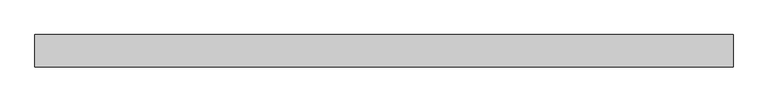
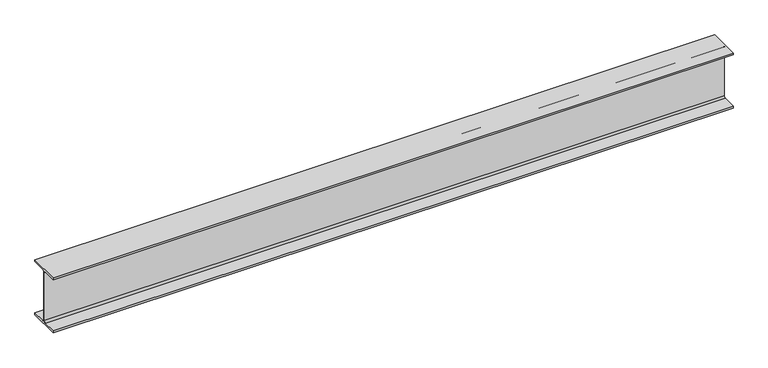
"""IFC4 building model written with IfcOpenShell, lengths in millimetres: beam geometry, Old_Steel Beam_H-KSD3502 : H_SB_ASB_H-200×200x8x12."""

from ifc_helpers import new_model, si_unit, point, frame, frame_2d, origin, place, context, project, spatial, polyline, circle_curve, trimmed, segment, composite_curve, outline, extrude, source, transform, mapped, element, save


def beam_b41741f2(model_context):
    return source(origin(), model_context, "Body", "SweptSolid", [
        extrude(outline(composite_curve([segment(polyline([(82.5, -141.5), (82.5, -151.7), (-82.5, -151.7), (-82.5, -141.5), (-11.9, -141.5)]), True, "CONTINUOUS"), segment(trimmed(circle_curve(frame_2d((-11.9, -132.6)), 8.9), [point((-11.9, -141.5))], [point((-3.0, -132.6))], True, "CARTESIAN"), True, "CONTINUOUS"), segment(polyline([(-3.0, -132.6), (-3.0, 132.6)]), True, "CONTINUOUS"), segment(trimmed(circle_curve(frame_2d((-11.9, 132.6)), 8.9), [point((-3.0, 132.6))], [point((-11.9, 141.5))], True, "CARTESIAN"), True, "CONTINUOUS"), segment(polyline([(-11.9, 141.5), (-82.5, 141.5), (-82.5, 151.7), (82.5, 151.7), (82.5, 141.5), (11.9, 141.5)]), True, "CONTINUOUS"), segment(trimmed(circle_curve(frame_2d((11.9, 132.6)), 8.9), [point((11.9, 141.5))], [point((3.0, 132.6))], True, "CARTESIAN"), True, "CONTINUOUS"), segment(polyline([(3.0, 132.6), (3.0, -132.6)]), True, "CONTINUOUS"), segment(trimmed(circle_curve(frame_2d((11.9, -132.6)), 8.9), [point((3.0, -132.6))], [point((11.9, -141.5))], True, "CARTESIAN"), True, "CONTINUOUS"), segment(polyline([(11.9, -141.5), (82.5, -141.5)]), True, "CONTINUOUS")], self_intersect=False)), frame((-1826.0344939, 0.0, 0.0), z_axis=(1.0, 0.0, 0.0), x_axis=(0.0, 1.0, 0.0)), (0.0, 0.0, 1.0), 3548.8457304),
    ])


if __name__ == "__main__":
    model = new_model("IFC4")
    model_context = context("Model", 3, world=origin())
    ifc_project = project(units=[si_unit("LENGTHUNIT", "METRE", prefix="MILLI")], contexts=[model_context])
    site = spatial("IfcSite", under=ifc_project)
    building = spatial("IfcBuilding", under=site)
    placement = place(None, origin())
    beam_shape = beam_b41741f2(model_context)
    element("IfcBeam", 1, ObjectType="Old_Steel Beam_H-KSD3502 : H_SB_ASB_H-200×200x8x12", at=placement, inside=building, context=model_context, shape_type="MappedRepresentation", body=[
        mapped(beam_shape, transform((0.0, 0.0, 0.0), x_axis=(1.0, 0.0, 0.0), y_axis=(0.0, 1.0, 0.0), z_axis=(0.0, 0.0, 1.0))),
    ])
    save(model, "model.ifc")

# Revit data of these elements
# Type "Old_Steel Beam_H-KSD3502 : H_SB_ASB_H-200×200x8x12"
#   Width = 20.0 cm
#   Web Thickness = 0.8 cm
#   Web Fillet = 1.3 cm
#   Warping Constant = 141376.0 cm⁶
#   Torsional Moment of Inertia = 26.2485 cm⁴
#   Torsional Modulus = 1.0 cm³
#   Section Area = 63.53 cm²
#   Plastic Modulus weak axis = 244.0 cm³
#   Plastic Modulus strong axis = 525.0 cm³
#   Perimeter = 1.16 m²/m
#   Nominal Weight = 49.90 kgf/m
#   Moment of Inertia weak axis = 1600.00 cm⁴
#   Moment of Inertia strong axis = 4720.00 cm⁴
#   Height = 20.0 cm
#   Flange Thickness = 1.2 cm
#   Elastic Modulus weak axis = 160.0 cm³
#   Elastic Modulus strong axis = 472.0 cm³
#   Centroid Vertical = 10.0 cm
#   Centroid Horizontal = 10.0 cm
#   Length [instance default] = 1.5240 m
#   Structural Material [instance default] = Steel, 45-345
#   Assembly Code = ""
# Element 1 (IfcBeam, "Old_Steel Beam_H-KSD3502 : H_SB_ASB_H-200×200x8x12")
#   Structural Material = none
# Materials
#   "Steel, 45-345": class "Metal", colour RGB 189 187 185, transparency 0, Description = "Steel 345 MPa", Cost = 0
